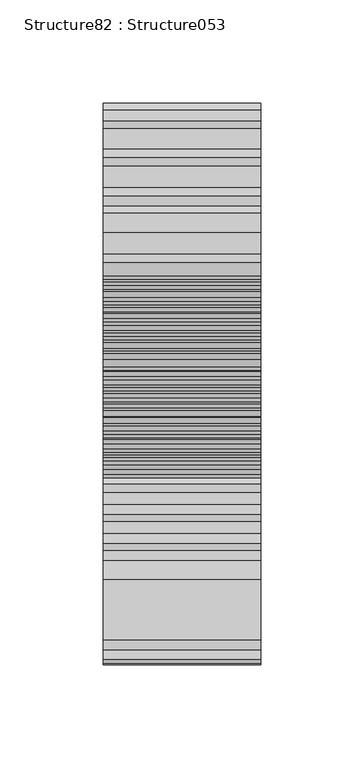
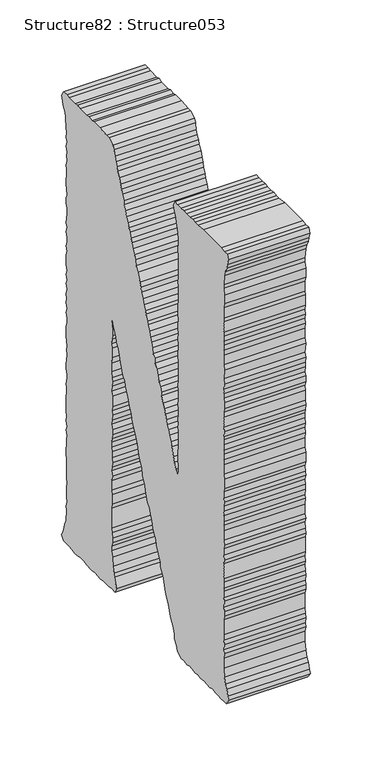
"""IFC4 building model written with IfcOpenShell, lengths in millimetres: proxy geometry, Structure82 : Structure053."""

import ifcopenshell
import ifcopenshell.guid

model = None  # the IFC model being written
_history = None  # IfcOwnerHistory: only IFC2X3 demands one
_inside = {}  # id of a spatial element -> (the spatial element, [elements in it])
_under = {}  # id of a project, library or spatial element -> (it, [spatial elements below it])
_declared = {}  # id of a project -> (the project, [libraries it declares])
_typed = {}  # id of a type object -> (the type object, [elements of that type])
_made_of = {}  # id of a material, layer set ... -> (it, [elements and type objects made of it])


def new_model(schema):
    """Start an empty IFC model of exactly this schema.

    Asked for "IFC4X3", IfcOpenShell would pick the latest addendum, in which some entities
    have other attributes; the version numbers below select the first issue.
    IFC2X3 requires an IfcOwnerHistory on every rooted entity: one is made here for all.
    """
    global model, _history
    if schema == "IFC4X3":
        model = ifcopenshell.file(schema_version=(4, 3, 0, 0))
    else:
        model = ifcopenshell.file(schema=schema)
    _inside.clear()
    _under.clear()
    _declared.clear()
    _typed.clear()
    _made_of.clear()
    _history = None
    if model.schema == "IFC2X3":
        org = make("IfcOrganization", Name="unknown")
        user = make(
            "IfcPersonAndOrganization",
            ThePerson=make("IfcPerson", FamilyName="unknown"),
            TheOrganization=org,
        )
        app = make(
            "IfcApplication",
            ApplicationDeveloper=org,
            Version="unknown",
            ApplicationFullName="unknown",
            ApplicationIdentifier="unknown",
        )
        _history = make(
            "IfcOwnerHistory",
            OwningUser=user,
            OwningApplication=app,
            ChangeAction="ADDED",
            CreationDate=0,
        )
    return model


def make(cls, **values):
    """One entity of the class cls with the attributes given. An attribute that is None is left unset."""
    return model.create_entity(
        cls, **{name: value for name, value in values.items() if value is not None}
    )


def rooted(cls, **values):
    """An entity with a GlobalId (a new one), such as an element, a storey or a relation."""
    return make(cls, GlobalId=ifcopenshell.guid.new(), OwnerHistory=_history, **values)


def si_unit(unit_type, name, prefix=None):
    """IfcSIUnit, for example si_unit("LENGTHUNIT", "METRE", prefix="MILLI")."""
    return make("IfcSIUnit", UnitType=unit_type, Prefix=prefix, Name=name)


def assignment(units):
    """IfcUnitAssignment: the units of a project."""
    return None if units is None else make("IfcUnitAssignment", Units=units)


def point(xyz):
    """IfcCartesianPoint."""
    return None if xyz is None else make("IfcCartesianPoint", Coordinates=xyz)


def direction(xyz):
    """IfcDirection."""
    return None if xyz is None else make("IfcDirection", DirectionRatios=xyz)


def frame(location, z_axis=None, x_axis=None):
    """IfcAxis2Placement3D, a coordinate frame: its origin and axes. An axis left out is left unset."""
    return make(
        "IfcAxis2Placement3D",
        Location=point(location),
        Axis=direction(z_axis),
        RefDirection=direction(x_axis),
    )


def origin():
    """The frame at (0, 0, 0) with its axes left unset."""
    return frame((0.0, 0.0, 0.0))


def place(relative_to, where):
    """IfcLocalPlacement: puts the frame where relative to a parent placement (None: the world)."""
    return make(
        "IfcLocalPlacement", PlacementRelTo=relative_to, RelativePlacement=where
    )


def context(
    kind, dimensions, precision=None, world=None, true_north=None, identifier=None
):
    """IfcGeometricRepresentationContext, for example the 3D "Model" context."""
    return make(
        "IfcGeometricRepresentationContext",
        ContextIdentifier=identifier,
        ContextType=kind,
        CoordinateSpaceDimension=dimensions,
        Precision=precision,
        WorldCoordinateSystem=world,
        TrueNorth=true_north,
    )


def project(units=None, contexts=None):
    """IfcProject with its units and contexts."""
    return rooted(
        "IfcProject",
        Name="project",
        RepresentationContexts=contexts,
        UnitsInContext=assignment(units),
    )


def spatial(cls, under=None, at=None, **own):
    """A site, building, storey or space (cls), placed at a placement, below another one or the project."""
    s = rooted(cls, ObjectPlacement=at, **own)
    if under is not None:
        _under.setdefault(under.id(), (under, []))[1].append(s)
    return s


def polyline(points):
    """IfcPolyline through the points."""
    return make("IfcPolyline", Points=[point(p) for p in points])


def outline(outer, holes=None, kind="AREA"):
    """IfcArbitraryClosedProfileDef: a profile drawn as a closed curve; with holes, ...WithVoids."""
    if holes is None:
        return make("IfcArbitraryClosedProfileDef", ProfileType=kind, OuterCurve=outer)
    return make(
        "IfcArbitraryProfileDefWithVoids",
        ProfileType=kind,
        OuterCurve=outer,
        InnerCurves=holes,
    )


def extrude(swept, where, along, depth):
    """IfcExtrudedAreaSolid: the profile swept, set in the frame where, extruded along a direction by depth."""
    return make(
        "IfcExtrudedAreaSolid",
        SweptArea=swept,
        Position=where,
        ExtrudedDirection=direction(along),
        Depth=depth,
    )


def shape(context_of_items, identifier, shape_type, items):
    """IfcShapeRepresentation: the items that make up one representation, for example the "Body"."""
    return make(
        "IfcShapeRepresentation",
        ContextOfItems=context_of_items,
        RepresentationIdentifier=identifier,
        RepresentationType=shape_type,
        Items=items,
    )


def source(mapping_origin, context_of_items, identifier, shape_type, items):
    """IfcRepresentationMap: a shape defined once, which mapped items show again and again."""
    return make(
        "IfcRepresentationMap",
        MappingOrigin=mapping_origin,
        MappedRepresentation=shape(context_of_items, identifier, shape_type, items),
    )


def transform(
    local_origin,
    x_axis=None,
    y_axis=None,
    z_axis=None,
    scale=None,
    scale2=None,
    scale3=None,
    uniform=True,
):
    """IfcCartesianTransformationOperator3D, or its non-uniform kind. x_axis, y_axis, z_axis: its Axis1, 2, 3."""
    if uniform:
        return make(
            "IfcCartesianTransformationOperator3D",
            Axis1=direction(x_axis),
            Axis2=direction(y_axis),
            LocalOrigin=point(local_origin),
            Scale=scale,
            Axis3=direction(z_axis),
        )
    return make(
        "IfcCartesianTransformationOperator3DnonUniform",
        Axis1=direction(x_axis),
        Axis2=direction(y_axis),
        LocalOrigin=point(local_origin),
        Scale=scale,
        Axis3=direction(z_axis),
        Scale2=scale2,
        Scale3=scale3,
    )


def mapped(mapping_source, mapping_target):
    """IfcMappedItem: shows the shape of a source again, moved by a transform."""
    return make(
        "IfcMappedItem", MappingSource=mapping_source, MappingTarget=mapping_target
    )


def made_of(thing, what):
    """Note that an element or type object is made of a material, layer set ...; save() writes the relation."""
    if what is not None:
        _made_of.setdefault(what.id(), (what, []))[1].append(thing)
    return thing


def element(
    cls,
    number,
    at=None,
    inside=None,
    cuts=None,
    type_object=None,
    material=None,
    context=None,
    identifier="Body",
    shape_type=None,
    held_by="IfcProductDefinitionShape",
    body=None,
    shapes=None,
    **own,
):
    """One element of the class cls, such as IfcWall. Its Tag is "e" and its number.

    at: its placement. inside: the storey or other place that contains it. cuts: it is an
    opening in that element (IfcRelVoidsElement). A single representation is given by context,
    identifier, shape_type and body (its items); several are given by shapes. held_by: the class
    of the entity that holds the representations. save() writes the other relations.
    """
    e = rooted(cls, Tag="e%d" % number, ObjectPlacement=at, **own)
    if body is not None:
        shapes = [shape(context, identifier, shape_type, body)]
    if shapes is not None:
        e.Representation = make(held_by, Representations=shapes)
    if inside is not None:
        _inside.setdefault(inside.id(), (inside, []))[1].append(e)
    if cuts is not None:
        rooted(
            "IfcRelVoidsElement", RelatingBuildingElement=cuts, RelatedOpeningElement=e
        )
    if type_object is not None:
        _typed.setdefault(type_object.id(), (type_object, []))[1].append(e)
    return made_of(e, material)


def aggregate(whole, parts):
    """IfcRelAggregates: a whole, such as a stair, and the parts it consists of."""
    return rooted("IfcRelAggregates", RelatingObject=whole, RelatedObjects=parts)


def save(model, path):
    """Write the relations noted so far, then the file.

    IfcRelAggregates (storeys below a building ...), IfcRelContainedInSpatialStructure (elements
    in a storey), IfcRelDefinesByType, IfcRelAssociatesMaterial and IfcRelDeclares: one each for
    every whole, place, type object, material and project.
    """
    for whole, parts in _under.values():
        aggregate(whole, parts)
    for where, things in _inside.values():
        rooted(
            "IfcRelContainedInSpatialStructure",
            RelatedElements=things,
            RelatingStructure=where,
        )
    for kind, things in _typed.values():
        rooted("IfcRelDefinesByType", RelatedObjects=things, RelatingType=kind)
    for what, things in _made_of.values():
        rooted("IfcRelAssociatesMaterial", RelatedObjects=things, RelatingMaterial=what)
    for by, libraries in _declared.values():
        rooted("IfcRelDeclares", RelatingContext=by, RelatedDefinitions=libraries)
    model.write(path)


def structure82_structure053_e44646d9(model_context):
    return source(origin(), model_context, "Body", "SweptSolid", [
        extrude(outline(polyline([(276597.3447251, 3575.0851816), (276598.5048541, 3583.2863152), (276599.685843, 3589.1527492), (276599.685843, 3593.8285667), (276598.5048541, 3597.9540049), (276598.5048541, 3602.0280957), (276599.1065808, 3607.3393366), (276599.685843, 3611.4134274), (276599.685843, 3631.3410106), (276599.1065808, 3635.4407751), (276599.1065808, 3644.8245022), (276599.685843, 3648.9258713), (276599.685843, 3658.3015753), (276598.5048541, 3663.5598643), (276599.685843, 3668.2437048), (276599.1065808, 3672.3691429), (276598.5048541, 3677.0449605), (276599.1065808, 3681.7271964), (276599.1065808, 3687.587212), (276599.685843, 3691.6869765), (276599.685843, 3696.3884676), (276599.1065808, 3700.4705815), (276598.5048541, 3704.5879966), (276598.5048541, 3709.8559132), (276599.685843, 3714.5301261), (276599.1065808, 3718.6571688), (276598.5048541, 3723.9154578), (276599.1065808, 3728.0152223), (276598.5048541, 3732.7167134), (276598.5048541, 3742.6748889), (276599.685843, 3747.3587295), (276599.1065808, 3752.6170184), (276598.5048541, 3757.3185096), (276599.1065808, 3760.818152), (276599.685843, 3766.684586), (276599.685843, 3774.8857196), (276599.1065808, 3780.7441306), (276599.1065808, 3790.1294623), (276599.685843, 3794.2292268), (276599.1065808, 3798.9050443), (276598.5048541, 3803.0064134), (276598.5048541, 3808.8888934), (276599.1065808, 3812.9726119), (276599.685843, 3818.2309008), (276598.5048541, 3817.6741031), (276596.1637362, 3812.9726119), (276594.4259495, 3808.290376), (276592.6656984, 3804.7730829), (276591.4847095, 3800.6717138), (276588.5418648, 3795.960595), (276586.8040782, 3790.7039107), (276585.6230892, 3787.2042683), (276584.4645648, 3782.5027771), (276582.6802446, 3777.8285642), (276580.9199935, 3773.7015215), (276578.0236824, 3770.2018791), (276576.8426934, 3766.1021146), (276574.479111, 3760.2437036), (276573.343051, 3757.3185096), (276570.9810732, 3752.6170184), (276569.8000843, 3748.5429276), (276567.4589664, 3743.8414364), (276566.8797041, 3739.1592005), (276563.9609286, 3733.8736333), (276562.7799396, 3730.3563402), (276560.4163572, 3725.6741043), (276558.6561061, 3722.1568112), (276556.9183194, 3716.8985223), (276556.3390572, 3712.7971532), (276554.5788061, 3708.087639), (276552.2152236, 3703.4134261), (276550.477437, 3700.4705815), (276549.2964481, 3694.6298211), (276547.5361969, 3691.0868544), (276545.195079, 3686.4030139), (276544.6158168, 3681.7271964), (276541.0953145, 3672.9435914), (276538.1524698, 3668.8261762), (276536.3922187, 3664.1423357), (276535.2561587, 3660.6250426), (276532.8941809, 3655.9428067), (276532.3149187, 3651.8590883), (276529.9513363, 3647.1575971), (276527.6342874, 3643.6579547), (276527.0325607, 3638.3563415), (276524.6930473, 3634.2822506), (276522.9311916, 3630.1824862), (276520.5916782, 3625.472972), (276520.012416, 3621.3732075), (276517.071176, 3616.69739), (276515.3093202, 3613.1720739), (276513.5490691, 3607.3393366), (276512.9922714, 3603.7963698), (276511.2095558, 3599.7126514), (276507.6874489, 3591.5131224), (276505.3704, 3586.8116312), (276504.1894111, 3581.5276686), (276501.8482931, 3577.4535778), (276499.4863153, 3573.3265351), (276497.7485286, 3568.0682461), (276497.1692664, 3563.9412034), (276494.2264218, 3559.2669905), (276492.4661706, 3555.1848766), (276486.6045504, 3551.0658569), (276482.5047859, 3551.0658569), (276477.2224279, 3550.4833855), (276472.5434012, 3551.6675836), (276469.0212944, 3551.6675836), (276463.7614008, 3550.4833855), (276459.0823741, 3551.6675836), (276454.9585406, 3550.4833855), (276449.0969203, 3551.0658569), (276445.5988825, 3551.0658569), (276439.7147978, 3550.4833855), (276436.21676, 3551.6675836), (276430.934402, 3551.0658569), (276426.833033, 3551.0658569), (276420.9954818, 3550.4833855), (276416.8716482, 3551.0658569), (276412.7718838, 3551.0658569), (276409.2497769, 3556.3417965), (276410.4307658, 3559.8671125), (276412.1910169, 3565.7094775), (276414.5545994, 3569.2524442), (276416.292386, 3575.0851816), (276417.4509105, 3583.2863152), (276417.4509105, 3593.2541183), (276416.292386, 3598.5284533), (276416.8716482, 3602.0280957), (276416.292386, 3607.3393366), (276416.8716482, 3611.4134274), (276417.4509105, 3616.69739), (276417.4509105, 3631.3410106), (276416.292386, 3635.4407751), (276416.292386, 3640.114988), (276416.8716482, 3644.2420307), (276416.292386, 3650.1004418), (276416.8716482, 3653.6000842), (276417.4509105, 3659.4584952), (276416.8716482, 3662.9854159), (276417.4509105, 3668.2437048), (276416.8716482, 3672.3691429), (276416.8716482, 3687.0127636), (276416.292386, 3691.0868544), (276416.8716482, 3695.786741), (276417.4509105, 3701.6547796), (276416.292386, 3705.7545441), (276417.4509105, 3709.8559132), (276417.4509105, 3719.2316172), (276416.8716482, 3725.0996559), (276417.4509105, 3728.5992983), (276416.8716482, 3734.47536), (276416.8716482, 3739.1592005), (276417.4509105, 3743.8414364), (276416.292386, 3748.5429276), (276416.8716482, 3752.04257), (276417.4509105, 3757.8753073), (276416.292386, 3762.0023501), (276416.292386, 3771.3860772), (276417.4509105, 3775.4874463), (276417.4509105, 3784.8438951), (276416.8716482, 3790.1294623), (276417.4509105, 3795.4037973), (276416.8716482, 3799.5051664), (276417.4509105, 3804.7730829), (276417.4509105, 3809.4729695), (276416.8716482, 3812.9726119), (276416.292386, 3818.2309008), (276416.8716482, 3822.348316), (276416.8716482, 3832.3161191), (276417.4509105, 3836.9919366), (276416.292386, 3841.0900965), (276416.292386, 3846.9757858), (276417.4509105, 3850.4754282), (276416.8716482, 3855.7353217), (276416.8716482, 3859.8591552), (276416.292386, 3865.1190488), (276417.4509105, 3869.8189354), (276416.292386, 3879.1769888), (276417.4509105, 3883.8881076), (276417.4509105, 3893.246161), (276416.8716482, 3898.5301236), (276417.4509105, 3903.2059411), (276416.8716482, 3907.3313793), (276417.4509105, 3912.0071968), (276416.8716482, 3916.6653636), (276416.8716482, 3926.6492128), (276417.4509105, 3930.1745289), (276417.4509105, 3940.1166583), (276416.292386, 3944.8165449), (276416.292386, 3953.5937315), (276417.4509105, 3959.4617701), (276417.4509105, 3962.9774586), (276416.292386, 3972.9372387), (276414.5545994, 3977.6194746), (276412.1910169, 3982.8793681), (276411.6117547, 3986.4046842), (276409.8515036, 3992.2614906), (276411.6117547, 3996.9645864), (276416.292386, 3996.390138), (276420.9954818, 3997.5486624), (276450.2795138, 3997.5486624), (276459.6616363, 3996.390138), (276464.340663, 3996.390138), (276467.8627699, 3997.5486624), (276472.5434012, 3996.390138), (276478.4034168, 3996.390138), (276481.9255237, 3997.5486624), (276486.6045504, 3996.9645864), (276492.4661706, 3996.9645864), (276496.5675397, 3997.5486624), (276499.4863153, 3992.2614906), (276497.7485286, 3987.5792547), (276495.4090153, 3982.3225704), (276494.2264218, 3978.2035506), (276492.4661706, 3972.9372387), (276490.728384, 3964.1343784), (276490.728384, 3959.4617701), (276491.864444, 3954.7506513), (276490.728384, 3944.235678), (276491.2851817, 3940.718385), (276490.728384, 3936.0345445), (276491.2851817, 3930.7329312), (276491.2851817, 3925.4746423), (276491.864444, 3921.3748778), (276490.728384, 3916.6653636), (276491.2851817, 3912.5896682), (276491.2851817, 3903.2059411), (276491.864444, 3897.3475301), (276491.864444, 3887.9621984), (276490.728384, 3884.4609514), (276491.864444, 3878.5784713), (276491.864444, 3873.9203044), (276491.2851817, 3870.4030114), (276491.864444, 3864.5446004), (276490.728384, 3859.8591552), (276490.728384, 3856.3161885), (276491.864444, 3850.4754282), (276491.864444, 3846.9757858), (276490.728384, 3842.2758992), (276490.728384, 3832.8921721), (276491.2851817, 3828.2163546), (276490.728384, 3823.5341187), (276491.864444, 3818.2309008), (276491.2851817, 3813.5743386), (276490.728384, 3810.0474179), (276491.2851817, 3804.1890069), (276491.864444, 3800.0876378), (276490.728384, 3794.8309535), (276490.728384, 3790.1294623), (276491.864444, 3785.4456218), (276490.728384, 3780.7441306), (276491.864444, 3777.2444882), (276491.2851817, 3772.5606477), (276491.2851817, 3767.2590344), (276490.728384, 3762.5848215), (276490.728384, 3757.3185096), (276491.864444, 3753.8012165), (276491.864444, 3744.4158848), (276490.728384, 3738.5574738), (276490.728384, 3735.0578314), (276491.864444, 3730.3563402), (276493.0454329, 3729.1737467), (276494.8072886, 3733.2991849), (276497.1692664, 3739.1592005), (276498.9070531, 3743.2332913), (276501.2465664, 3752.04257), (276503.6101489, 3755.559863), (276505.9271978, 3760.2437036), (276507.6874489, 3764.9435901), (276509.4493046, 3768.4432325), (276510.6302935, 3773.11905), (276511.8112824, 3777.8285642), (276513.5490691, 3781.9299333), (276515.8885825, 3786.0280932), (276518.2521649, 3791.8865042), (276518.8314271, 3795.4037973), (276520.5916782, 3799.5051664), (276522.3294649, 3803.5872802), (276524.6930473, 3808.290376), (276525.8740362, 3813.5743386), (276528.7928118, 3817.6741031), (276529.372074, 3822.348316), (276532.3149187, 3825.2911606), (276533.4734431, 3830.5574726), (276535.2561587, 3834.6588416), (276536.3922187, 3838.7586061), (276538.1524698, 3844.0345457), (276540.5160523, 3848.7167816), (276541.6970412, 3851.6612309), (276543.4348278, 3857.5019912), (276544.6158168, 3860.4432313), (276546.9569347, 3864.5446004), (276548.7171858, 3869.8189354), (276551.0566992, 3874.5043805), (276551.6359614, 3879.1769888), (276553.3962126, 3883.2863809), (276556.9183194, 3890.905043), (276559.837095, 3895.5888836), (276561.0180839, 3900.8648231), (276562.2006774, 3904.9645876), (276565.119453, 3909.0627475), (276566.2779774, 3914.3499193), (276568.0382286, 3917.8479571), (276569.8000843, 3922.5494483), (276570.9810732, 3926.6492128), (276573.343051, 3930.1745289), (276575.0808377, 3934.8503464), (276576.8426934, 3939.5325823), (276579.1822068, 3944.235678), (276579.7839335, 3947.7337158), (276582.1009824, 3952.9920048), (276583.2819713, 3957.1190475), (276585.043827, 3961.2204166), (276586.8040782, 3966.5043792), (276589.7228537, 3971.1785921), (276590.9038426, 3974.7055128), (276592.6656984, 3978.8036727), (276594.4259495, 3982.8793681), (276595.6069384, 3988.7634528), (276597.3447251, 3992.2614906), (276603.7856075, 3995.7803883), (276607.8869766, 3995.7803883), (276618.4276236, 3996.9645864), (276627.809746, 3996.9645864), (276631.3318529, 3995.7803883), (276636.0124842, 3996.9645864), (276640.1347132, 3995.7803883), (276650.6545002, 3995.7803883), (276654.7767292, 3996.9645864), (276658.8556338, 3995.7803883), (276668.839483, 3995.7803883), (276672.3375208, 3996.9645864), (276677.6198788, 3996.390138), (276681.1195212, 3991.0788971), (276679.3576655, 3986.4046842), (276678.2216055, 3982.8793681), (276675.2803654, 3977.6194746), (276674.0993765, 3973.5197101), (276673.5201143, 3962.9774586), (276672.9183876, 3959.4617701), (276673.5201143, 3953.5937315), (276672.3375208, 3950.0940891), (276673.5201143, 3944.8165449), (276672.3375208, 3940.1166583), (276672.9183876, 3936.0345445), (276672.3375208, 3931.3346579), (276673.5201143, 3926.6492128), (276672.9183876, 3921.9733953), (276672.9183876, 3916.0909152), (276673.5201143, 3912.5896682), (276673.5201143, 3907.3313793), (276672.9183876, 3902.6314927), (276672.3375208, 3897.3475301), (276673.5201143, 3893.822214), (276673.5201143, 3888.5623205), (276672.3375208, 3884.4609514), (276672.3375208, 3879.1769888), (276672.9183876, 3873.9203044), (276673.5201143, 3869.2444869), (276672.3375208, 3865.7015202), (276673.5201143, 3861.0192843), (276672.3375208, 3855.1769193), (276672.3375208, 3851.0595042), (276673.5201143, 3846.3772683), (276672.3375208, 3841.6741725), (276673.5201143, 3837.6000817), (276673.5201143, 3828.2163546), (276672.3375208, 3822.348316), (276673.5201143, 3818.2309008), (276672.3375208, 3812.9726119), (276673.5201143, 3809.4729695), (276672.3375208, 3804.1890069), (276673.5201143, 3798.9050443), (276672.9183876, 3794.2292268), (276673.5201143, 3790.7039107), (276672.3375208, 3784.8438951), (276673.5201143, 3780.7441306), (276672.3375208, 3776.0618947), (276672.3375208, 3771.3860772), (276673.5201143, 3766.684586), (276673.5201143, 3757.3185096), (276672.9183876, 3752.04257), (276672.3375208, 3747.9428055), (276672.9183876, 3743.8414364), (276672.3375208, 3739.1592005), (276672.9183876, 3733.8736333), (276673.5201143, 3729.7738688), (276673.5201143, 3725.0996559), (276672.3375208, 3719.2316172), (276672.3375208, 3715.7143242), (276673.5201143, 3709.8559132), (276672.9183876, 3706.3289925), (276672.9183876, 3701.6547796), (276673.5201143, 3696.9709391), (276673.5201143, 3682.3289231), (276672.9183876, 3678.2018803), (276673.5201143, 3672.9435914), (276672.3375208, 3667.6853024), (276673.5201143, 3664.1423357), (276672.3375208, 3659.4584952), (276672.9183876, 3654.7842823), (276672.9183876, 3649.5003197), (276673.5201143, 3644.8245022), (276673.5201143, 3640.114988), (276672.9183876, 3635.4407751), (276672.9183876, 3616.69739), (276672.3375208, 3612.0135494), (276672.9183876, 3607.8961343), (276672.9183876, 3597.9540049), (276672.3375208, 3593.2541183), (276673.5201143, 3589.1527492), (276672.9183876, 3584.4689087), (276673.5201143, 3574.5107332), (276675.8596277, 3569.2524442), (276677.0406166, 3565.1254015), (276678.2216055, 3561.025637), (276681.1195212, 3555.7416744), (276677.6198788, 3551.6675836), (276668.2377563, 3551.6675836), (276658.8556338, 3550.4833855), (276654.197467, 3550.4833855), (276650.6545002, 3551.6675836), (276644.8153445, 3551.6675836), (276640.7139754, 3550.4833855), (276631.9111151, 3550.4833855), (276626.6287571, 3551.0658569), (276622.5514571, 3550.4833855), (276617.2690991, 3550.4833855), (276613.7485968, 3551.0658569), (276603.7856075, 3551.0658569), (276599.1065808, 3551.6675836), (276594.4259495, 3551.0658569), (276591.4847095, 3556.3417965), (276595.0052117, 3565.7094775), (276595.6069384, 3569.2524442), (276597.3447251, 3575.0851816)])), frame((-59031.6926606, 0.0, 0.0), z_axis=(1.0, 0.0, 0.0), x_axis=(0.0, 1.0, 0.0)), (0.0, 0.0, 1.0), 76.2),
    ])


if __name__ == "__main__":
    model = new_model("IFC4")
    model_context = context("Model", 3, world=origin())
    ifc_project = project(units=[si_unit("LENGTHUNIT", "METRE", prefix="MILLI")], contexts=[model_context])
    site = spatial("IfcSite", under=ifc_project)
    building = spatial("IfcBuilding", under=site)
    placement = place(None, origin())
    structure82_structure053_shape = structure82_structure053_e44646d9(model_context)
    element("IfcBuildingElementProxy", 1, Name="Structure82 : Structure053", ObjectType="Structure82 : Structure053", at=placement, inside=building, context=model_context, shape_type="MappedRepresentation", body=[
        mapped(structure82_structure053_shape, transform((0.0, 0.0, 0.0), x_axis=(1.0, 0.0, 0.0), y_axis=(0.0, 1.0, 0.0), z_axis=(0.0, 0.0, 1.0))),
    ])
    save(model, "model.ifc")

# Revit data of these elements
# Type "Structure82 : Structure053"
#   NameOverride = "Structure053"
# Element 1 (IfcBuildingElementProxy, "Structure82 : Structure053")
#   Materials on its faces: "BRUSHED ALUM. LETTERING"
# Materials
#   "BRUSHED ALUM. LETTERING": class "Unassigned", colour RGB 169 181 186, transparency 0, Cost = 0
